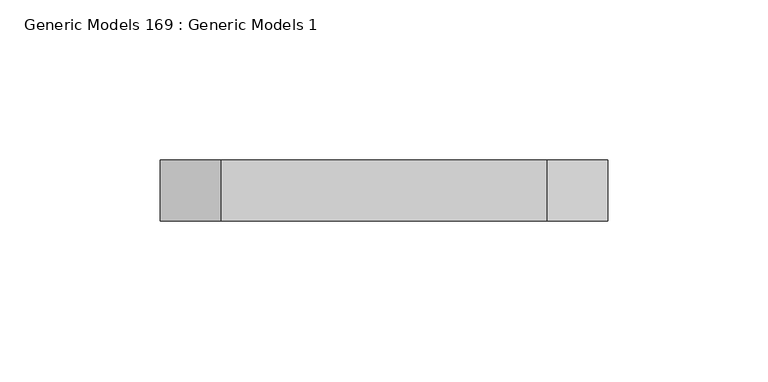
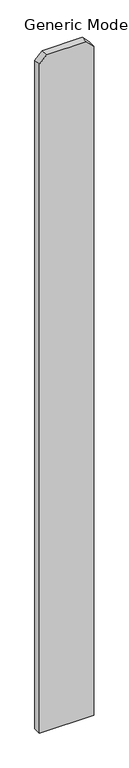
"""IFC4 building model written with IfcOpenShell, lengths in millimetres: proxy geometry, Generic Models 169 : Generic Models 1."""

import ifcopenshell
import ifcopenshell.guid

model = None  # the IFC model being written
_history = None  # IfcOwnerHistory: only IFC2X3 demands one
_inside = {}  # id of a spatial element -> (the spatial element, [elements in it])
_under = {}  # id of a project, library or spatial element -> (it, [spatial elements below it])
_declared = {}  # id of a project -> (the project, [libraries it declares])
_typed = {}  # id of a type object -> (the type object, [elements of that type])
_made_of = {}  # id of a material, layer set ... -> (it, [elements and type objects made of it])


def new_model(schema):
    """Start an empty IFC model of exactly this schema.

    Asked for "IFC4X3", IfcOpenShell would pick the latest addendum, in which some entities
    have other attributes; the version numbers below select the first issue.
    IFC2X3 requires an IfcOwnerHistory on every rooted entity: one is made here for all.
    """
    global model, _history
    if schema == "IFC4X3":
        model = ifcopenshell.file(schema_version=(4, 3, 0, 0))
    else:
        model = ifcopenshell.file(schema=schema)
    _inside.clear()
    _under.clear()
    _declared.clear()
    _typed.clear()
    _made_of.clear()
    _history = None
    if model.schema == "IFC2X3":
        org = make("IfcOrganization", Name="unknown")
        user = make(
            "IfcPersonAndOrganization",
            ThePerson=make("IfcPerson", FamilyName="unknown"),
            TheOrganization=org,
        )
        app = make(
            "IfcApplication",
            ApplicationDeveloper=org,
            Version="unknown",
            ApplicationFullName="unknown",
            ApplicationIdentifier="unknown",
        )
        _history = make(
            "IfcOwnerHistory",
            OwningUser=user,
            OwningApplication=app,
            ChangeAction="ADDED",
            CreationDate=0,
        )
    return model


def make(cls, **values):
    """One entity of the class cls with the attributes given. An attribute that is None is left unset."""
    return model.create_entity(
        cls, **{name: value for name, value in values.items() if value is not None}
    )


def rooted(cls, **values):
    """An entity with a GlobalId (a new one), such as an element, a storey or a relation."""
    return make(cls, GlobalId=ifcopenshell.guid.new(), OwnerHistory=_history, **values)


def si_unit(unit_type, name, prefix=None):
    """IfcSIUnit, for example si_unit("LENGTHUNIT", "METRE", prefix="MILLI")."""
    return make("IfcSIUnit", UnitType=unit_type, Prefix=prefix, Name=name)


def assignment(units):
    """IfcUnitAssignment: the units of a project."""
    return None if units is None else make("IfcUnitAssignment", Units=units)


def point(xyz):
    """IfcCartesianPoint."""
    return None if xyz is None else make("IfcCartesianPoint", Coordinates=xyz)


def direction(xyz):
    """IfcDirection."""
    return None if xyz is None else make("IfcDirection", DirectionRatios=xyz)


def frame(location, z_axis=None, x_axis=None):
    """IfcAxis2Placement3D, a coordinate frame: its origin and axes. An axis left out is left unset."""
    return make(
        "IfcAxis2Placement3D",
        Location=point(location),
        Axis=direction(z_axis),
        RefDirection=direction(x_axis),
    )


def origin():
    """The frame at (0, 0, 0) with its axes left unset."""
    return frame((0.0, 0.0, 0.0))


def place(relative_to, where):
    """IfcLocalPlacement: puts the frame where relative to a parent placement (None: the world)."""
    return make(
        "IfcLocalPlacement", PlacementRelTo=relative_to, RelativePlacement=where
    )


def context(
    kind, dimensions, precision=None, world=None, true_north=None, identifier=None
):
    """IfcGeometricRepresentationContext, for example the 3D "Model" context."""
    return make(
        "IfcGeometricRepresentationContext",
        ContextIdentifier=identifier,
        ContextType=kind,
        CoordinateSpaceDimension=dimensions,
        Precision=precision,
        WorldCoordinateSystem=world,
        TrueNorth=true_north,
    )


def project(units=None, contexts=None):
    """IfcProject with its units and contexts."""
    return rooted(
        "IfcProject",
        Name="project",
        RepresentationContexts=contexts,
        UnitsInContext=assignment(units),
    )


def spatial(cls, under=None, at=None, **own):
    """A site, building, storey or space (cls), placed at a placement, below another one or the project."""
    s = rooted(cls, ObjectPlacement=at, **own)
    if under is not None:
        _under.setdefault(under.id(), (under, []))[1].append(s)
    return s


def polyline(points):
    """IfcPolyline through the points."""
    return make("IfcPolyline", Points=[point(p) for p in points])


def outline(outer, holes=None, kind="AREA"):
    """IfcArbitraryClosedProfileDef: a profile drawn as a closed curve; with holes, ...WithVoids."""
    if holes is None:
        return make("IfcArbitraryClosedProfileDef", ProfileType=kind, OuterCurve=outer)
    return make(
        "IfcArbitraryProfileDefWithVoids",
        ProfileType=kind,
        OuterCurve=outer,
        InnerCurves=holes,
    )


def extrude(swept, where, along, depth):
    """IfcExtrudedAreaSolid: the profile swept, set in the frame where, extruded along a direction by depth."""
    return make(
        "IfcExtrudedAreaSolid",
        SweptArea=swept,
        Position=where,
        ExtrudedDirection=direction(along),
        Depth=depth,
    )


def shape(context_of_items, identifier, shape_type, items):
    """IfcShapeRepresentation: the items that make up one representation, for example the "Body"."""
    return make(
        "IfcShapeRepresentation",
        ContextOfItems=context_of_items,
        RepresentationIdentifier=identifier,
        RepresentationType=shape_type,
        Items=items,
    )


def source(mapping_origin, context_of_items, identifier, shape_type, items):
    """IfcRepresentationMap: a shape defined once, which mapped items show again and again."""
    return make(
        "IfcRepresentationMap",
        MappingOrigin=mapping_origin,
        MappedRepresentation=shape(context_of_items, identifier, shape_type, items),
    )


def transform(
    local_origin,
    x_axis=None,
    y_axis=None,
    z_axis=None,
    scale=None,
    scale2=None,
    scale3=None,
    uniform=True,
):
    """IfcCartesianTransformationOperator3D, or its non-uniform kind. x_axis, y_axis, z_axis: its Axis1, 2, 3."""
    if uniform:
        return make(
            "IfcCartesianTransformationOperator3D",
            Axis1=direction(x_axis),
            Axis2=direction(y_axis),
            LocalOrigin=point(local_origin),
            Scale=scale,
            Axis3=direction(z_axis),
        )
    return make(
        "IfcCartesianTransformationOperator3DnonUniform",
        Axis1=direction(x_axis),
        Axis2=direction(y_axis),
        LocalOrigin=point(local_origin),
        Scale=scale,
        Axis3=direction(z_axis),
        Scale2=scale2,
        Scale3=scale3,
    )


def mapped(mapping_source, mapping_target):
    """IfcMappedItem: shows the shape of a source again, moved by a transform."""
    return make(
        "IfcMappedItem", MappingSource=mapping_source, MappingTarget=mapping_target
    )


def made_of(thing, what):
    """Note that an element or type object is made of a material, layer set ...; save() writes the relation."""
    if what is not None:
        _made_of.setdefault(what.id(), (what, []))[1].append(thing)
    return thing


def element(
    cls,
    number,
    at=None,
    inside=None,
    cuts=None,
    type_object=None,
    material=None,
    context=None,
    identifier="Body",
    shape_type=None,
    held_by="IfcProductDefinitionShape",
    body=None,
    shapes=None,
    **own,
):
    """One element of the class cls, such as IfcWall. Its Tag is "e" and its number.

    at: its placement. inside: the storey or other place that contains it. cuts: it is an
    opening in that element (IfcRelVoidsElement). A single representation is given by context,
    identifier, shape_type and body (its items); several are given by shapes. held_by: the class
    of the entity that holds the representations. save() writes the other relations.
    """
    e = rooted(cls, Tag="e%d" % number, ObjectPlacement=at, **own)
    if body is not None:
        shapes = [shape(context, identifier, shape_type, body)]
    if shapes is not None:
        e.Representation = make(held_by, Representations=shapes)
    if inside is not None:
        _inside.setdefault(inside.id(), (inside, []))[1].append(e)
    if cuts is not None:
        rooted(
            "IfcRelVoidsElement", RelatingBuildingElement=cuts, RelatedOpeningElement=e
        )
    if type_object is not None:
        _typed.setdefault(type_object.id(), (type_object, []))[1].append(e)
    return made_of(e, material)


def aggregate(whole, parts):
    """IfcRelAggregates: a whole, such as a stair, and the parts it consists of."""
    return rooted("IfcRelAggregates", RelatingObject=whole, RelatedObjects=parts)


def save(model, path):
    """Write the relations noted so far, then the file.

    IfcRelAggregates (storeys below a building ...), IfcRelContainedInSpatialStructure (elements
    in a storey), IfcRelDefinesByType, IfcRelAssociatesMaterial and IfcRelDeclares: one each for
    every whole, place, type object, material and project.
    """
    for whole, parts in _under.values():
        aggregate(whole, parts)
    for where, things in _inside.values():
        rooted(
            "IfcRelContainedInSpatialStructure",
            RelatedElements=things,
            RelatingStructure=where,
        )
    for kind, things in _typed.values():
        rooted("IfcRelDefinesByType", RelatedObjects=things, RelatingType=kind)
    for what, things in _made_of.values():
        rooted("IfcRelAssociatesMaterial", RelatedObjects=things, RelatingMaterial=what)
    for by, libraries in _declared.values():
        rooted("IfcRelDeclares", RelatingContext=by, RelatedDefinitions=libraries)
    model.write(path)


def generic_models_169_generic_models_1_bddc7243(model_context):
    return source(origin(), model_context, "Body", "SweptSolid", [
        extrude(outline(polyline([(76.2, 55751.4125), (1885.95, 55751.4125), (1905.0, 55732.3625), (1905.0, 55630.7625), (1885.95, 55611.7125), (76.2, 55611.7125), (76.2, 55751.4125)])), frame((0.0, 547.6875, 0.0), z_axis=(0.0, 1.0, 0.0), x_axis=(0.0, 0.0, 1.0)), (0.0, 0.0, 1.0), 19.05),
    ])


if __name__ == "__main__":
    model = new_model("IFC4")
    model_context = context("Model", 3, world=origin())
    ifc_project = project(units=[si_unit("LENGTHUNIT", "METRE", prefix="MILLI")], contexts=[model_context])
    site = spatial("IfcSite", under=ifc_project)
    building = spatial("IfcBuilding", under=site)
    placement = place(None, origin())
    generic_models_169_generic_models_1_shape = generic_models_169_generic_models_1_bddc7243(model_context)
    element("IfcBuildingElementProxy", 1, Name="Generic Models 169 : Generic Models 1", ObjectType="Generic Models 169 : Generic Models 1", at=placement, inside=building, context=model_context, shape_type="MappedRepresentation", body=[
        mapped(generic_models_169_generic_models_1_shape, transform((0.0, 0.0, 0.0), x_axis=(1.0, 0.0, 0.0), y_axis=(0.0, 1.0, 0.0), z_axis=(0.0, 0.0, 1.0))),
    ])
    save(model, "model.ifc")

# Revit data of these elements
# Element 1 (IfcBuildingElementProxy, "Generic Models 169 : Generic Models 1")
#   Materials on its faces: "VERTICAL 1X6 CEDAR PLANKS W/ CLEAR WOOD SEALER"
# Materials
#   "VERTICAL 1X6 CEDAR PLANKS W/ CLEAR WOOD SEALER": class "Wood", colour RGB 234 198 147, transparency 0, Description = "Pinus Echinata", Cost = 0
